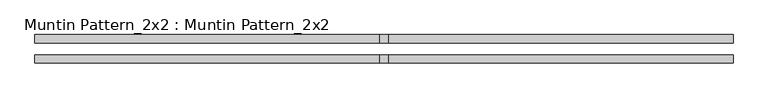
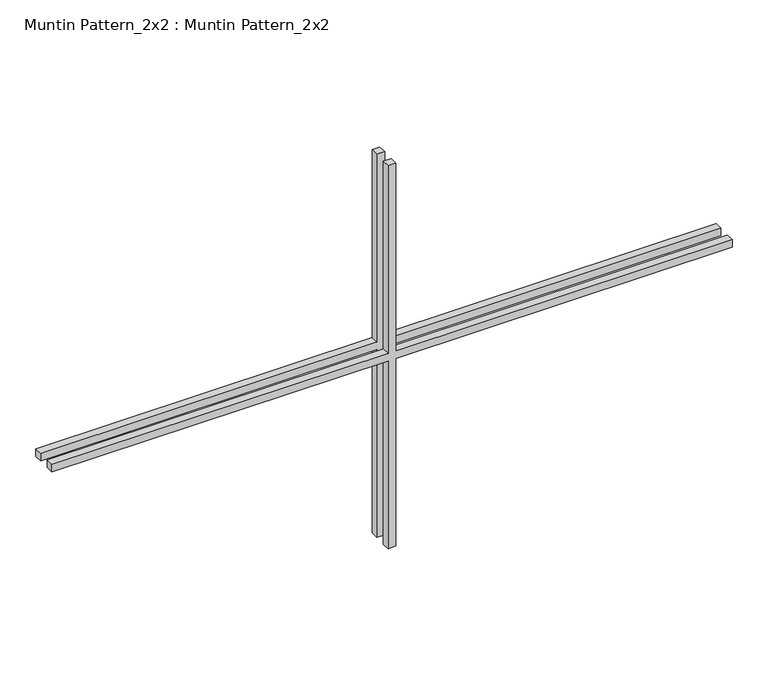
"""IFC4 building model written with IfcOpenShell, lengths in millimetres: proxy geometry, Muntin Pattern_2x2 : Muntin Pattern_2x2."""

import ifcopenshell
import ifcopenshell.guid

model = None  # the IFC model being written
_history = None  # IfcOwnerHistory: only IFC2X3 demands one
_inside = {}  # id of a spatial element -> (the spatial element, [elements in it])
_under = {}  # id of a project, library or spatial element -> (it, [spatial elements below it])
_declared = {}  # id of a project -> (the project, [libraries it declares])
_typed = {}  # id of a type object -> (the type object, [elements of that type])
_made_of = {}  # id of a material, layer set ... -> (it, [elements and type objects made of it])


def new_model(schema):
    """Start an empty IFC model of exactly this schema.

    Asked for "IFC4X3", IfcOpenShell would pick the latest addendum, in which some entities
    have other attributes; the version numbers below select the first issue.
    IFC2X3 requires an IfcOwnerHistory on every rooted entity: one is made here for all.
    """
    global model, _history
    if schema == "IFC4X3":
        model = ifcopenshell.file(schema_version=(4, 3, 0, 0))
    else:
        model = ifcopenshell.file(schema=schema)
    _inside.clear()
    _under.clear()
    _declared.clear()
    _typed.clear()
    _made_of.clear()
    _history = None
    if model.schema == "IFC2X3":
        org = make("IfcOrganization", Name="unknown")
        user = make(
            "IfcPersonAndOrganization",
            ThePerson=make("IfcPerson", FamilyName="unknown"),
            TheOrganization=org,
        )
        app = make(
            "IfcApplication",
            ApplicationDeveloper=org,
            Version="unknown",
            ApplicationFullName="unknown",
            ApplicationIdentifier="unknown",
        )
        _history = make(
            "IfcOwnerHistory",
            OwningUser=user,
            OwningApplication=app,
            ChangeAction="ADDED",
            CreationDate=0,
        )
    return model


def make(cls, **values):
    """One entity of the class cls with the attributes given. An attribute that is None is left unset."""
    return model.create_entity(
        cls, **{name: value for name, value in values.items() if value is not None}
    )


def rooted(cls, **values):
    """An entity with a GlobalId (a new one), such as an element, a storey or a relation."""
    return make(cls, GlobalId=ifcopenshell.guid.new(), OwnerHistory=_history, **values)


def si_unit(unit_type, name, prefix=None):
    """IfcSIUnit, for example si_unit("LENGTHUNIT", "METRE", prefix="MILLI")."""
    return make("IfcSIUnit", UnitType=unit_type, Prefix=prefix, Name=name)


def assignment(units):
    """IfcUnitAssignment: the units of a project."""
    return None if units is None else make("IfcUnitAssignment", Units=units)


def point(xyz):
    """IfcCartesianPoint."""
    return None if xyz is None else make("IfcCartesianPoint", Coordinates=xyz)


def direction(xyz):
    """IfcDirection."""
    return None if xyz is None else make("IfcDirection", DirectionRatios=xyz)


def frame(location, z_axis=None, x_axis=None):
    """IfcAxis2Placement3D, a coordinate frame: its origin and axes. An axis left out is left unset."""
    return make(
        "IfcAxis2Placement3D",
        Location=point(location),
        Axis=direction(z_axis),
        RefDirection=direction(x_axis),
    )


def origin():
    """The frame at (0, 0, 0) with its axes left unset."""
    return frame((0.0, 0.0, 0.0))


def place(relative_to, where):
    """IfcLocalPlacement: puts the frame where relative to a parent placement (None: the world)."""
    return make(
        "IfcLocalPlacement", PlacementRelTo=relative_to, RelativePlacement=where
    )


def context(
    kind, dimensions, precision=None, world=None, true_north=None, identifier=None
):
    """IfcGeometricRepresentationContext, for example the 3D "Model" context."""
    return make(
        "IfcGeometricRepresentationContext",
        ContextIdentifier=identifier,
        ContextType=kind,
        CoordinateSpaceDimension=dimensions,
        Precision=precision,
        WorldCoordinateSystem=world,
        TrueNorth=true_north,
    )


def project(units=None, contexts=None):
    """IfcProject with its units and contexts."""
    return rooted(
        "IfcProject",
        Name="project",
        RepresentationContexts=contexts,
        UnitsInContext=assignment(units),
    )


def spatial(cls, under=None, at=None, **own):
    """A site, building, storey or space (cls), placed at a placement, below another one or the project."""
    s = rooted(cls, ObjectPlacement=at, **own)
    if under is not None:
        _under.setdefault(under.id(), (under, []))[1].append(s)
    return s


def polyline(points):
    """IfcPolyline through the points."""
    return make("IfcPolyline", Points=[point(p) for p in points])


def outline(outer, holes=None, kind="AREA"):
    """IfcArbitraryClosedProfileDef: a profile drawn as a closed curve; with holes, ...WithVoids."""
    if holes is None:
        return make("IfcArbitraryClosedProfileDef", ProfileType=kind, OuterCurve=outer)
    return make(
        "IfcArbitraryProfileDefWithVoids",
        ProfileType=kind,
        OuterCurve=outer,
        InnerCurves=holes,
    )


def extrude(swept, where, along, depth):
    """IfcExtrudedAreaSolid: the profile swept, set in the frame where, extruded along a direction by depth."""
    return make(
        "IfcExtrudedAreaSolid",
        SweptArea=swept,
        Position=where,
        ExtrudedDirection=direction(along),
        Depth=depth,
    )


def shape(context_of_items, identifier, shape_type, items):
    """IfcShapeRepresentation: the items that make up one representation, for example the "Body"."""
    return make(
        "IfcShapeRepresentation",
        ContextOfItems=context_of_items,
        RepresentationIdentifier=identifier,
        RepresentationType=shape_type,
        Items=items,
    )


def source(mapping_origin, context_of_items, identifier, shape_type, items):
    """IfcRepresentationMap: a shape defined once, which mapped items show again and again."""
    return make(
        "IfcRepresentationMap",
        MappingOrigin=mapping_origin,
        MappedRepresentation=shape(context_of_items, identifier, shape_type, items),
    )


def transform(
    local_origin,
    x_axis=None,
    y_axis=None,
    z_axis=None,
    scale=None,
    scale2=None,
    scale3=None,
    uniform=True,
):
    """IfcCartesianTransformationOperator3D, or its non-uniform kind. x_axis, y_axis, z_axis: its Axis1, 2, 3."""
    if uniform:
        return make(
            "IfcCartesianTransformationOperator3D",
            Axis1=direction(x_axis),
            Axis2=direction(y_axis),
            LocalOrigin=point(local_origin),
            Scale=scale,
            Axis3=direction(z_axis),
        )
    return make(
        "IfcCartesianTransformationOperator3DnonUniform",
        Axis1=direction(x_axis),
        Axis2=direction(y_axis),
        LocalOrigin=point(local_origin),
        Scale=scale,
        Axis3=direction(z_axis),
        Scale2=scale2,
        Scale3=scale3,
    )


def mapped(mapping_source, mapping_target):
    """IfcMappedItem: shows the shape of a source again, moved by a transform."""
    return make(
        "IfcMappedItem", MappingSource=mapping_source, MappingTarget=mapping_target
    )


def made_of(thing, what):
    """Note that an element or type object is made of a material, layer set ...; save() writes the relation."""
    if what is not None:
        _made_of.setdefault(what.id(), (what, []))[1].append(thing)
    return thing


def element(
    cls,
    number,
    at=None,
    inside=None,
    cuts=None,
    type_object=None,
    material=None,
    context=None,
    identifier="Body",
    shape_type=None,
    held_by="IfcProductDefinitionShape",
    body=None,
    shapes=None,
    **own,
):
    """One element of the class cls, such as IfcWall. Its Tag is "e" and its number.

    at: its placement. inside: the storey or other place that contains it. cuts: it is an
    opening in that element (IfcRelVoidsElement). A single representation is given by context,
    identifier, shape_type and body (its items); several are given by shapes. held_by: the class
    of the entity that holds the representations. save() writes the other relations.
    """
    e = rooted(cls, Tag="e%d" % number, ObjectPlacement=at, **own)
    if body is not None:
        shapes = [shape(context, identifier, shape_type, body)]
    if shapes is not None:
        e.Representation = make(held_by, Representations=shapes)
    if inside is not None:
        _inside.setdefault(inside.id(), (inside, []))[1].append(e)
    if cuts is not None:
        rooted(
            "IfcRelVoidsElement", RelatingBuildingElement=cuts, RelatedOpeningElement=e
        )
    if type_object is not None:
        _typed.setdefault(type_object.id(), (type_object, []))[1].append(e)
    return made_of(e, material)


def aggregate(whole, parts):
    """IfcRelAggregates: a whole, such as a stair, and the parts it consists of."""
    return rooted("IfcRelAggregates", RelatingObject=whole, RelatedObjects=parts)


def save(model, path):
    """Write the relations noted so far, then the file.

    IfcRelAggregates (storeys below a building ...), IfcRelContainedInSpatialStructure (elements
    in a storey), IfcRelDefinesByType, IfcRelAssociatesMaterial and IfcRelDeclares: one each for
    every whole, place, type object, material and project.
    """
    for whole, parts in _under.values():
        aggregate(whole, parts)
    for where, things in _inside.values():
        rooted(
            "IfcRelContainedInSpatialStructure",
            RelatedElements=things,
            RelatingStructure=where,
        )
    for kind, things in _typed.values():
        rooted("IfcRelDefinesByType", RelatedObjects=things, RelatingType=kind)
    for what, things in _made_of.values():
        rooted("IfcRelAssociatesMaterial", RelatedObjects=things, RelatingMaterial=what)
    for by, libraries in _declared.values():
        rooted("IfcRelDeclares", RelatingContext=by, RelatedDefinitions=libraries)
    model.write(path)


def muntin_pattern_2x2_muntin_pattern_2x2_d2a59152(model_context):
    return source(origin(), model_context, "Body", "SweptSolid", [
        extrude(outline(polyline([(331.7875, -6.35), (331.7875, -546.1), (319.0875, -546.1), (319.0875, -6.35), (0.0, -6.35), (0.0, 6.35), (319.0875, 6.35), (319.0875, 546.1), (331.7875, 546.1), (331.7875, 6.35), (650.875, 6.35), (650.875, -6.35), (331.7875, -6.35)])), frame((0.0, -22.225, 0.0), z_axis=(0.0, 1.0, 0.0), x_axis=(0.0, 0.0, 1.0)), (0.0, 0.0, 1.0), 12.7),
        extrude(outline(polyline([(331.7875, -6.35), (331.7875, -546.1), (319.0875, -546.1), (319.0875, -6.35), (0.0, -6.35), (0.0, 6.35), (319.0875, 6.35), (319.0875, 546.1), (331.7875, 546.1), (331.7875, 6.35), (650.875, 6.35), (650.875, -6.35), (331.7875, -6.35)])), frame((0.0, 9.525, 0.0), z_axis=(0.0, 1.0, 0.0), x_axis=(0.0, 0.0, 1.0)), (0.0, 0.0, 1.0), 12.7),
    ])


if __name__ == "__main__":
    model = new_model("IFC4")
    model_context = context("Model", 3, world=origin())
    ifc_project = project(units=[si_unit("LENGTHUNIT", "METRE", prefix="MILLI")], contexts=[model_context])
    site = spatial("IfcSite", under=ifc_project)
    building = spatial("IfcBuilding", under=site)
    placement = place(None, origin())
    muntin_pattern_2x2_muntin_pattern_2x2_shape = muntin_pattern_2x2_muntin_pattern_2x2_d2a59152(model_context)
    element("IfcBuildingElementProxy", 1, Name="Muntin Pattern_2x2 : Muntin Pattern_2x2", ObjectType="Muntin Pattern_2x2 : Muntin Pattern_2x2", at=placement, inside=building, context=model_context, shape_type="MappedRepresentation", body=[
        mapped(muntin_pattern_2x2_muntin_pattern_2x2_shape, transform((0.0, 0.0, 0.0), x_axis=(1.0, 0.0, 0.0), y_axis=(0.0, 1.0, 0.0), z_axis=(0.0, 0.0, 1.0))),
    ])
    save(model, "model.ifc")

# Revit data of these elements
# Type "Muntin Pattern_2x2 : Muntin Pattern_2x2"
#   Width [instance default] = 4' - 0"
#   Thickness = 0' - 0 1/2"
#   Height [instance default] = 4' - 0"
#   Distance = 0' - 0 3/4"
#   Interior Material [instance default] = none
#   Exterior Material [instance default] = none
# Element 1 (IfcBuildingElementProxy, "Muntin Pattern_2x2 : Muntin Pattern_2x2")
#   Width = 3' - 7"
#   Height = 2' - 1 5/8"
#   Interior Material = Wood - Stained
#   Exterior Material = Clad - White
#   Materials on its faces: "Clad - White", "Wood - Stained"
# Materials
#   "Clad - White": class "Wood", colour RGB 242 242 238, transparency 0, Cost = 0
#   "Wood - Stained": class "Wood", colour RGB 224 178 126, transparency 0, Cost = 0
